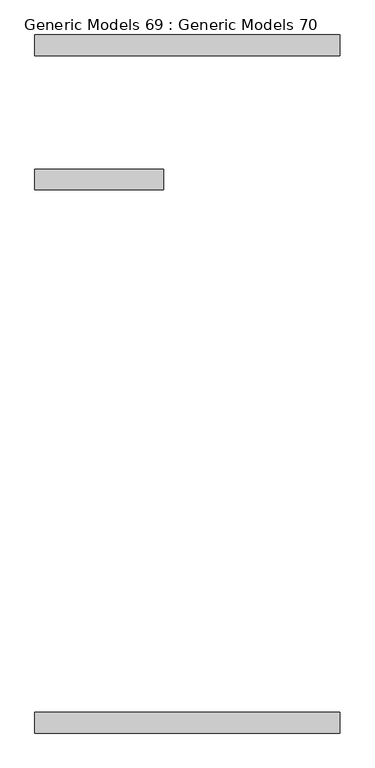
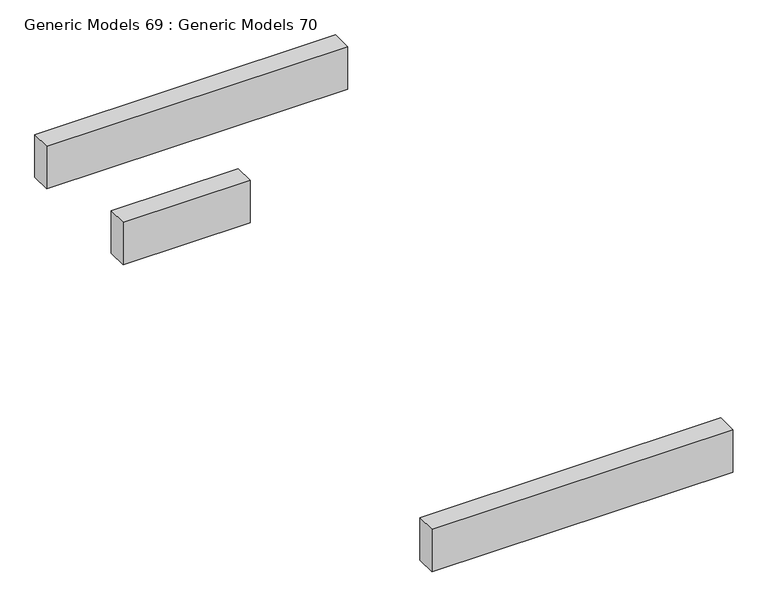
"""IFC4 building model written with IfcOpenShell, lengths in millimetres: proxy geometry, Generic Models 69 : Generic Models 70."""

import ifcopenshell
import ifcopenshell.guid

model = None  # the IFC model being written
_history = None  # IfcOwnerHistory: only IFC2X3 demands one
_inside = {}  # id of a spatial element -> (the spatial element, [elements in it])
_under = {}  # id of a project, library or spatial element -> (it, [spatial elements below it])
_declared = {}  # id of a project -> (the project, [libraries it declares])
_typed = {}  # id of a type object -> (the type object, [elements of that type])
_made_of = {}  # id of a material, layer set ... -> (it, [elements and type objects made of it])


def new_model(schema):
    """Start an empty IFC model of exactly this schema.

    Asked for "IFC4X3", IfcOpenShell would pick the latest addendum, in which some entities
    have other attributes; the version numbers below select the first issue.
    IFC2X3 requires an IfcOwnerHistory on every rooted entity: one is made here for all.
    """
    global model, _history
    if schema == "IFC4X3":
        model = ifcopenshell.file(schema_version=(4, 3, 0, 0))
    else:
        model = ifcopenshell.file(schema=schema)
    _inside.clear()
    _under.clear()
    _declared.clear()
    _typed.clear()
    _made_of.clear()
    _history = None
    if model.schema == "IFC2X3":
        org = make("IfcOrganization", Name="unknown")
        user = make(
            "IfcPersonAndOrganization",
            ThePerson=make("IfcPerson", FamilyName="unknown"),
            TheOrganization=org,
        )
        app = make(
            "IfcApplication",
            ApplicationDeveloper=org,
            Version="unknown",
            ApplicationFullName="unknown",
            ApplicationIdentifier="unknown",
        )
        _history = make(
            "IfcOwnerHistory",
            OwningUser=user,
            OwningApplication=app,
            ChangeAction="ADDED",
            CreationDate=0,
        )
    return model


def make(cls, **values):
    """One entity of the class cls with the attributes given. An attribute that is None is left unset."""
    return model.create_entity(
        cls, **{name: value for name, value in values.items() if value is not None}
    )


def rooted(cls, **values):
    """An entity with a GlobalId (a new one), such as an element, a storey or a relation."""
    return make(cls, GlobalId=ifcopenshell.guid.new(), OwnerHistory=_history, **values)


def si_unit(unit_type, name, prefix=None):
    """IfcSIUnit, for example si_unit("LENGTHUNIT", "METRE", prefix="MILLI")."""
    return make("IfcSIUnit", UnitType=unit_type, Prefix=prefix, Name=name)


def assignment(units):
    """IfcUnitAssignment: the units of a project."""
    return None if units is None else make("IfcUnitAssignment", Units=units)


def point(xyz):
    """IfcCartesianPoint."""
    return None if xyz is None else make("IfcCartesianPoint", Coordinates=xyz)


def direction(xyz):
    """IfcDirection."""
    return None if xyz is None else make("IfcDirection", DirectionRatios=xyz)


def frame(location, z_axis=None, x_axis=None):
    """IfcAxis2Placement3D, a coordinate frame: its origin and axes. An axis left out is left unset."""
    return make(
        "IfcAxis2Placement3D",
        Location=point(location),
        Axis=direction(z_axis),
        RefDirection=direction(x_axis),
    )


def origin():
    """The frame at (0, 0, 0) with its axes left unset."""
    return frame((0.0, 0.0, 0.0))


def place(relative_to, where):
    """IfcLocalPlacement: puts the frame where relative to a parent placement (None: the world)."""
    return make(
        "IfcLocalPlacement", PlacementRelTo=relative_to, RelativePlacement=where
    )


def context(
    kind, dimensions, precision=None, world=None, true_north=None, identifier=None
):
    """IfcGeometricRepresentationContext, for example the 3D "Model" context."""
    return make(
        "IfcGeometricRepresentationContext",
        ContextIdentifier=identifier,
        ContextType=kind,
        CoordinateSpaceDimension=dimensions,
        Precision=precision,
        WorldCoordinateSystem=world,
        TrueNorth=true_north,
    )


def project(units=None, contexts=None):
    """IfcProject with its units and contexts."""
    return rooted(
        "IfcProject",
        Name="project",
        RepresentationContexts=contexts,
        UnitsInContext=assignment(units),
    )


def spatial(cls, under=None, at=None, **own):
    """A site, building, storey or space (cls), placed at a placement, below another one or the project."""
    s = rooted(cls, ObjectPlacement=at, **own)
    if under is not None:
        _under.setdefault(under.id(), (under, []))[1].append(s)
    return s


def polyline(points):
    """IfcPolyline through the points."""
    return make("IfcPolyline", Points=[point(p) for p in points])


def outline(outer, holes=None, kind="AREA"):
    """IfcArbitraryClosedProfileDef: a profile drawn as a closed curve; with holes, ...WithVoids."""
    if holes is None:
        return make("IfcArbitraryClosedProfileDef", ProfileType=kind, OuterCurve=outer)
    return make(
        "IfcArbitraryProfileDefWithVoids",
        ProfileType=kind,
        OuterCurve=outer,
        InnerCurves=holes,
    )


def extrude(swept, where, along, depth):
    """IfcExtrudedAreaSolid: the profile swept, set in the frame where, extruded along a direction by depth."""
    return make(
        "IfcExtrudedAreaSolid",
        SweptArea=swept,
        Position=where,
        ExtrudedDirection=direction(along),
        Depth=depth,
    )


def shape(context_of_items, identifier, shape_type, items):
    """IfcShapeRepresentation: the items that make up one representation, for example the "Body"."""
    return make(
        "IfcShapeRepresentation",
        ContextOfItems=context_of_items,
        RepresentationIdentifier=identifier,
        RepresentationType=shape_type,
        Items=items,
    )


def source(mapping_origin, context_of_items, identifier, shape_type, items):
    """IfcRepresentationMap: a shape defined once, which mapped items show again and again."""
    return make(
        "IfcRepresentationMap",
        MappingOrigin=mapping_origin,
        MappedRepresentation=shape(context_of_items, identifier, shape_type, items),
    )


def transform(
    local_origin,
    x_axis=None,
    y_axis=None,
    z_axis=None,
    scale=None,
    scale2=None,
    scale3=None,
    uniform=True,
):
    """IfcCartesianTransformationOperator3D, or its non-uniform kind. x_axis, y_axis, z_axis: its Axis1, 2, 3."""
    if uniform:
        return make(
            "IfcCartesianTransformationOperator3D",
            Axis1=direction(x_axis),
            Axis2=direction(y_axis),
            LocalOrigin=point(local_origin),
            Scale=scale,
            Axis3=direction(z_axis),
        )
    return make(
        "IfcCartesianTransformationOperator3DnonUniform",
        Axis1=direction(x_axis),
        Axis2=direction(y_axis),
        LocalOrigin=point(local_origin),
        Scale=scale,
        Axis3=direction(z_axis),
        Scale2=scale2,
        Scale3=scale3,
    )


def mapped(mapping_source, mapping_target):
    """IfcMappedItem: shows the shape of a source again, moved by a transform."""
    return make(
        "IfcMappedItem", MappingSource=mapping_source, MappingTarget=mapping_target
    )


def made_of(thing, what):
    """Note that an element or type object is made of a material, layer set ...; save() writes the relation."""
    if what is not None:
        _made_of.setdefault(what.id(), (what, []))[1].append(thing)
    return thing


def element(
    cls,
    number,
    at=None,
    inside=None,
    cuts=None,
    type_object=None,
    material=None,
    context=None,
    identifier="Body",
    shape_type=None,
    held_by="IfcProductDefinitionShape",
    body=None,
    shapes=None,
    **own,
):
    """One element of the class cls, such as IfcWall. Its Tag is "e" and its number.

    at: its placement. inside: the storey or other place that contains it. cuts: it is an
    opening in that element (IfcRelVoidsElement). A single representation is given by context,
    identifier, shape_type and body (its items); several are given by shapes. held_by: the class
    of the entity that holds the representations. save() writes the other relations.
    """
    e = rooted(cls, Tag="e%d" % number, ObjectPlacement=at, **own)
    if body is not None:
        shapes = [shape(context, identifier, shape_type, body)]
    if shapes is not None:
        e.Representation = make(held_by, Representations=shapes)
    if inside is not None:
        _inside.setdefault(inside.id(), (inside, []))[1].append(e)
    if cuts is not None:
        rooted(
            "IfcRelVoidsElement", RelatingBuildingElement=cuts, RelatedOpeningElement=e
        )
    if type_object is not None:
        _typed.setdefault(type_object.id(), (type_object, []))[1].append(e)
    return made_of(e, material)


def aggregate(whole, parts):
    """IfcRelAggregates: a whole, such as a stair, and the parts it consists of."""
    return rooted("IfcRelAggregates", RelatingObject=whole, RelatedObjects=parts)


def save(model, path):
    """Write the relations noted so far, then the file.

    IfcRelAggregates (storeys below a building ...), IfcRelContainedInSpatialStructure (elements
    in a storey), IfcRelDefinesByType, IfcRelAssociatesMaterial and IfcRelDeclares: one each for
    every whole, place, type object, material and project.
    """
    for whole, parts in _under.values():
        aggregate(whole, parts)
    for where, things in _inside.values():
        rooted(
            "IfcRelContainedInSpatialStructure",
            RelatedElements=things,
            RelatingStructure=where,
        )
    for kind, things in _typed.values():
        rooted("IfcRelDefinesByType", RelatedObjects=things, RelatingType=kind)
    for what, things in _made_of.values():
        rooted("IfcRelAssociatesMaterial", RelatedObjects=things, RelatingMaterial=what)
    for by, libraries in _declared.values():
        rooted("IfcRelDeclares", RelatingContext=by, RelatedDefinitions=libraries)
    model.write(path)


def generic_models_69_generic_models_70_f7153194(model_context):
    return source(origin(), model_context, "Body", "SweptSolid", [
        extrude(outline(polyline([(33289.8715778, 36493.1457942), (33289.8715778, 36321.6957942), (30750.6865619, 36321.6957942), (30750.6865619, 36493.1457942), (33289.8715778, 36493.1457942)])), frame((0.0, 0.0, 268757.4), z_axis=(0.0, 0.0, 1.0), x_axis=(1.0, 0.0, 0.0)), (0.0, 0.0, 1.0), 381.0),
        extrude(outline(polyline([(31821.4221032, 35375.5457942), (31821.4221032, 35204.0957942), (30750.6865619, 35204.0957942), (30750.6865619, 35375.5457942), (31821.4221032, 35375.5457942)])), frame((0.0, 0.0, 268757.4), z_axis=(0.0, 0.0, 1.0), x_axis=(1.0, 0.0, 0.0)), (0.0, 0.0, 1.0), 381.0),
        extrude(outline(polyline([(33289.8715778, 30860.0656612), (33289.8715778, 30688.6156612), (30750.6865619, 30688.6156612), (30750.6865619, 30860.0656612), (33289.8715778, 30860.0656612)])), frame((0.0, 0.0, 268757.4), z_axis=(0.0, 0.0, 1.0), x_axis=(1.0, 0.0, 0.0)), (0.0, 0.0, 1.0), 381.0),
    ])


if __name__ == "__main__":
    model = new_model("IFC4")
    model_context = context("Model", 3, world=origin())
    ifc_project = project(units=[si_unit("LENGTHUNIT", "METRE", prefix="MILLI")], contexts=[model_context])
    site = spatial("IfcSite", under=ifc_project)
    building = spatial("IfcBuilding", under=site)
    placement = place(None, origin())
    generic_models_69_generic_models_70_shape = generic_models_69_generic_models_70_f7153194(model_context)
    element("IfcBuildingElementProxy", 1, Name="Generic Models 69 : Generic Models 70", ObjectType="Generic Models 69 : Generic Models 70", at=placement, inside=building, context=model_context, shape_type="MappedRepresentation", body=[
        mapped(generic_models_69_generic_models_70_shape, transform((0.0, 0.0, 0.0), x_axis=(1.0, 0.0, 0.0), y_axis=(0.0, 1.0, 0.0), z_axis=(0.0, 0.0, 1.0))),
    ])
    save(model, "model.ifc")

# Revit data of these elements
# Element 1 (IfcBuildingElementProxy, "Generic Models 69 : Generic Models 70")
#   Materials on its faces: "6 3/4\" x 15\" GLUELAM BEAM"
# Materials
#   "6 3/4\" x 15\" GLUELAM BEAM": class "Wood", colour RGB 112 64 44, transparency 0, Description = "Pinus Echinata", Cost = 0
